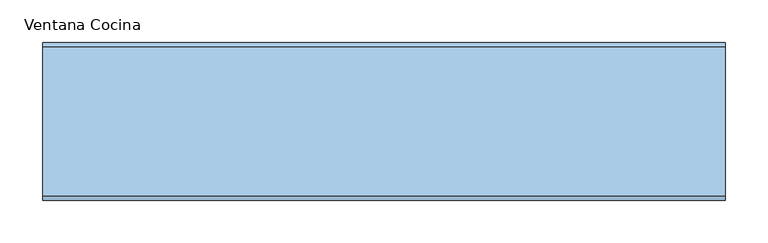
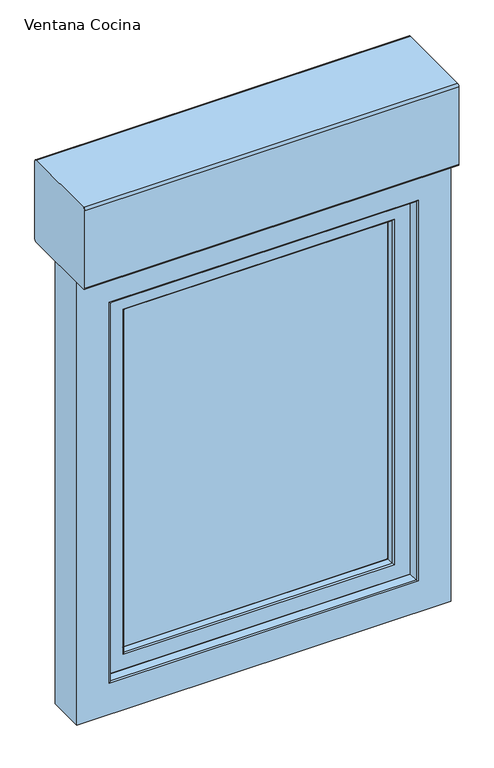
"""IFC4 building model written with IfcOpenShell, lengths in millimetres: window geometry, 2019_ES_Ventana_Replus_re80pvc301_10100_box_1-Hoja_con-Compacto : Ventana Cocina."""

from ifc_helpers import new_model, si_unit, point, frame, frame_2d, origin, place, context, project, spatial, polyline, circle_curve, ellipse_curve, trimmed, segment, composite_curve, outline, extrude, source, transform, mapped, element, save
from ifc_brep_helpers import plane_surface, cylinder_surface, advanced_brep


def ventana_cocina_4c5644c3(model_context):
    return source(origin(), model_context, "Body", "SolidModel", [
        extrude(outline(composite_curve([segment(trimmed(circle_curve(frame_2d((-55.0, 1815.0)), 5.0), [point((-55.0, 1810.0))], [point((-60.0, 1815.0))], False, "CARTESIAN"), True, "CONTINUOUS"), segment(polyline([(-60.0, 1815.0), (-60.0, 1990.0)]), True, "CONTINUOUS"), segment(trimmed(circle_curve(frame_2d((-55.0, 1990.0)), 5.0), [point((-60.0, 1990.0))], [point((-55.0, 1995.0))], False, "CARTESIAN"), True, "CONTINUOUS"), segment(polyline([(-55.0, 1995.0), (120.0, 1995.0)]), True, "CONTINUOUS"), segment(trimmed(circle_curve(frame_2d((120.0, 1990.0)), 5.0), [point((120.0, 1995.0))], [point((125.0, 1990.0))], False, "CARTESIAN"), True, "CONTINUOUS"), segment(polyline([(125.0, 1990.0), (125.0, 1815.0)]), True, "CONTINUOUS"), segment(trimmed(circle_curve(frame_2d((120.0, 1815.0)), 5.0), [point((125.0, 1815.0))], [point((120.0, 1810.0))], False, "CARTESIAN"), True, "CONTINUOUS"), segment(polyline([(120.0, 1810.0), (-55.0, 1810.0)]), True, "CONTINUOUS")], self_intersect=False)), frame((-400.0, 0.0, 0.0), z_axis=(1.0, 0.0, 0.0), x_axis=(0.0, 1.0, 0.0)), (0.0, 0.0, 1.0), 800.0),
        extrude(outline(polyline([(78.4999991, 1470.0), (118.4999991, 1470.0), (118.4999991, 1360.0), (98.4999991, 1360.0), (98.4999991, 1450.0), (78.4999991, 1450.0), (78.4999991, 1470.0)])), frame((-334.1999993, 0.0, 0.0), z_axis=(1.0, 0.0, 0.0), x_axis=(0.0, 1.0, 0.0)), (0.0, 0.0, 1.0), 12.0),
        extrude(outline(polyline([(-313.9687607, 78.4999991), (-313.9687607, 68.4999991), (-342.4312378, 68.4999991), (-342.4312378, 78.4999991), (-313.9687607, 78.4999991)])), frame((0.0, 0.0, 1435.217127), z_axis=(0.0, 0.0, 1.0), x_axis=(1.0, 0.0, 0.0)), (0.0, 0.0, 1.0), 49.565746),
        extrude(outline(polyline([(909.8, 297.1999993), (1707.2, 297.1999993), (1707.2, -297.1999993), (909.8, -297.1999993), (909.8, 297.1999993)]), holes=[polyline([(1699.2, 289.1999993), (917.8, 289.1999993), (917.8, -289.1999993), (1699.2, -289.1999993), (1699.2, 289.1999993)])]), frame((0.0, 10.9999999, 0.0), z_axis=(0.0, 1.0, 0.0), x_axis=(0.0, 0.0, 1.0)), (0.0, 0.0, 1.0), 16.0),
        extrude(outline(polyline([(909.8131934, 297.1868058), (1707.1868066, 297.1868058), (1707.1868066, -297.1868058), (909.8131934, -297.1868058), (909.8131934, 297.1868058)]), holes=[polyline([(1699.2, 289.1999993), (917.8, 289.1999993), (917.8, -289.1999993), (1699.2, -289.1999993), (1699.2, 289.1999993)])]), frame((0.0, 31.0000001, 0.0), z_axis=(0.0, 1.0, 0.0), x_axis=(0.0, 0.0, 1.0)), (0.0, 0.0, 1.0), 16.0),
        extrude(outline(polyline([(297.1999993, 6.9999997), (-297.1999993, 6.9999997), (-297.1999993, 10.9999999), (297.1999993, 10.9999999), (297.1999993, 6.9999997)])), frame((0.0, 0.0, 903.7946451), z_axis=(0.0, 0.0, 1.0), x_axis=(1.0, 0.0, 0.0)), (0.0, 0.0, 1.0), 809.4053549),
        extrude(outline(polyline([(297.1999993, 26.9999999), (-297.1999993, 26.9999999), (-297.1999993, 31.0000001), (297.1999993, 31.0000001), (297.1999993, 26.9999999)])), frame((0.0, 0.0, 903.7946451), z_axis=(0.0, 0.0, 1.0), x_axis=(1.0, 0.0, 0.0)), (0.0, 0.0, 1.0), 809.4053549),
        extrude(outline(polyline([(297.1999993, 47.0000001), (-297.1999993, 47.0000001), (-297.1999993, 51.0000003), (297.1999993, 51.0000003), (297.1999993, 47.0000001)])), frame((0.0, 0.0, 903.7946451), z_axis=(0.0, 0.0, 1.0), x_axis=(1.0, 0.0, 0.0)), (0.0, 0.0, 1.0), 809.4053549),
        advanced_brep(
        [(287.2913171, -9.2764571, 1697.2913178), (287.2913171, -9.2764571, 922.7086822), (290.1890946, -11.5, 919.8109047), (290.1890946, -11.5, 1700.1890953), (330.1999993, -11.5, 879.8), (330.1999993, -11.5, 1740.2), (-330.1999993, -11.5, 1740.2), (-330.1999993, -11.5, 879.8), (-290.1890946, -11.5, 919.8109047), (-290.1890946, -11.5, 1700.1890953), (-287.2913171, -9.2764571, 922.7086822), (284.1757968, 2.3508228, 1694.1757976), (284.1757968, 2.3508228, 925.8242024), (-284.1757968, 2.3508228, 925.8242024), (284.6739305, 3.0000033, 1694.6739313), (284.6739305, 3.0000033, 925.3260687), (-284.6739305, 3.0000033, 925.3260687), (291.1999993, 3.0000033, 1701.2), (291.1999993, 3.0000033, 918.8), (-291.1999993, 3.0000033, 918.8), (-291.1999993, 3.0000033, 1701.2), (-284.6739305, 3.0000033, 1694.6739313), (291.1999993, 6.9999997, 1701.2), (291.1999993, 6.9999997, 918.8), (-291.1999993, 6.9999997, 918.8), (311.8162192, 6.9999997, 1721.8162199), (311.8162192, 6.9999997, 898.1837801), (-311.8162192, 6.9999997, 898.1837801), (-311.8162192, 6.9999997, 1721.8162199), (-291.1999993, 6.9999997, 1701.2), (309.1999993, 25.6153717, 1719.2), (309.1999993, 25.6153717, 900.8), (-309.1999993, 25.6153717, 900.8), (309.1999993, 56.4999995, 1719.2), (309.1999993, 56.4999995, 900.8), (-309.1999993, 56.4999995, 900.8), (-309.1999993, 56.4999995, 1719.2), (297.1999993, 56.4999995, 1707.2), (297.1999993, 56.4999995, 912.8), (-297.1999993, 56.4999995, 912.8), (-297.1999993, 56.4999995, 1707.2), (297.1999993, 51.0000003, 1707.2), (297.1999993, 51.0000003, 912.8), (-297.1999993, 51.0000003, 912.8), (-297.1999993, 51.0000003, 1707.2), (286.007687, 51.0000003, 1696.0076877), (286.007687, 51.0000003, 923.9923123), (-286.007687, 51.0000003, 923.9923123), (-286.007687, 51.0000003, 1696.0076877), (285.4940999, 51.6693201, 1695.4941006), (285.4940999, 51.6693201, 924.5058994), (-285.4940999, 51.6693201, 924.5058994), (288.8993918, 64.3780426, 1698.8993925), (288.8993918, 64.3780426, 921.1006075), (-288.8993918, 64.3780426, 921.1006075), (292.6234971, 67.3403297, 1702.6234978), (292.6234971, 67.3403297, 917.3765022), (-292.6234971, 67.3403297, 917.3765022), (305.6488427, 67.7951848, 1715.6488434), (305.6488427, 67.7951848, 904.3511566), (-305.6488427, 67.7951848, 904.3511566), (306.1999993, 67.2629391, 1716.2), (306.1999993, 67.2629391, 903.8), (-306.1999993, 67.2629391, 903.8), (307.4370593, 68.4999991, 1717.43706), (307.4370593, 68.4999991, 902.56294), (-307.4370593, 68.4999991, 902.56294), (360.1999993, 68.4999991, 1770.2), (360.1999993, 68.4999991, 849.8), (-360.1999993, 68.4999991, 849.8), (-360.1999993, 68.4999991, 1770.2), (-307.4370593, 68.4999991, 1717.43706), (363.1999993, 65.4999991, 1773.2), (363.1999993, 65.4999991, 846.8), (-363.1999993, 65.4999991, 846.8), (363.1999993, 50.0, 1773.2), (363.1999993, 50.0, 846.8), (-363.1999993, 50.0, 846.8), (-363.1999993, 50.0, 1773.2), (343.1999993, 50.0, 1753.2), (343.1999993, 50.0, 866.8), (-343.1999993, 50.0, 866.8), (-343.1999993, 50.0, 1753.2), (343.1999993, 11.9999991, 1753.2), (343.1999993, 11.9999991, 866.8), (-343.1999993, 11.9999991, 866.8), (-343.1999993, 11.9999991, 1753.2), (330.1999993, 11.9999991, 1740.2), (330.1999993, 11.9999991, 879.8), (-330.1999993, 11.9999991, 879.8), (-330.1999993, 11.9999991, 1740.2), (-287.2913171, -9.2764571, 1697.2913178), (-284.1757968, 2.3508228, 1694.1757976), (-309.1999993, 25.6153717, 1719.2), (-285.4940999, 51.6693201, 1695.4941006), (-288.8993918, 64.3780426, 1698.8993925), (-292.6234971, 67.3403297, 1702.6234978), (-305.6488427, 67.7951848, 1715.6488434), (-306.1999993, 67.2629391, 1716.2), (-363.1999993, 65.4999991, 1773.2)],
        [
            (0, 1),
            (1, 2, ellipse_curve(frame((290.1890946, -8.5, 919.8109047), z_axis=(0.7071067811865475, 0.0, 0.7071067811865475), x_axis=(-0.7071067811865474, 0.0, 0.7071067811865476)), 4.2426407, 3.0)),
            (2, 3),
            (3, 0, ellipse_curve(frame((290.1890946, -8.5, 1700.1890953), z_axis=(0.7071067811865475, 0.0, -0.7071067811865475), x_axis=(0.7071067811865474, 0.0, 0.7071067811865476)), 4.2426407, 3.0)),
            (4, 5),
            (5, 6),
            (6, 7),
            (7, 4),
            (2, 8),
            (8, 9),
            (9, 3),
            (1, 10),
            (10, 8, ellipse_curve(frame((-290.1890946, -8.5, 919.8109047), z_axis=(0.7071067811865475, 0.0, -0.7071067811865475), x_axis=(0.7071067811865476, 0.0, 0.7071067811865474)), 4.2426407, 3.0)),
            (11, 12),
            (12, 1),
            (0, 11),
            (12, 13),
            (13, 10),
            (14, 15),
            (15, 12, ellipse_curve(frame((284.6739305, 2.4842973, 925.3260687), z_axis=(0.7071067811865475, 0.0, 0.7071067811865475), x_axis=(-0.7071067811865474, 0.0, 0.7071067811865476)), 0.7293184, 0.515706)),
            (11, 14, ellipse_curve(frame((284.6739305, 2.4842973, 1694.6739313), z_axis=(0.7071067811865475, 0.0, -0.7071067811865475), x_axis=(0.7071067811865474, 0.0, 0.7071067811865476)), 0.7293184, 0.515706)),
            (15, 16),
            (16, 13, ellipse_curve(frame((-284.6739305, 2.4842973, 925.3260687), z_axis=(0.7071067811865475, 0.0, -0.7071067811865475), x_axis=(0.7071067811865476, 0.0, 0.7071067811865474)), 0.7293184, 0.515706)),
            (17, 18),
            (18, 19),
            (19, 20),
            (20, 17),
            (14, 21),
            (21, 16),
            (22, 23),
            (23, 18),
            (17, 22),
            (23, 24),
            (24, 19),
            (25, 26),
            (26, 27),
            (27, 28),
            (28, 25),
            (22, 29),
            (29, 24),
            (30, 31),
            (31, 26),
            (25, 30),
            (31, 32),
            (32, 27),
            (33, 34),
            (34, 31),
            (30, 33),
            (34, 35),
            (35, 32),
            (33, 36),
            (36, 35),
            (37, 38),
            (38, 39),
            (39, 40),
            (40, 37),
            (41, 42),
            (42, 38),
            (37, 41),
            (42, 43),
            (43, 39),
            (41, 44),
            (44, 43),
            (45, 46),
            (46, 47),
            (47, 48),
            (48, 45),
            (49, 50),
            (50, 46, ellipse_curve(frame((286.007687, 51.5317048, 923.9923123), z_axis=(0.7071067811865475, 0.0, 0.7071067811865475), x_axis=(-0.7071067811865474, 0.0, 0.7071067811865476)), 0.7519437, 0.5317045)),
            (45, 49, ellipse_curve(frame((286.007687, 51.5317048, 1696.0076877), z_axis=(0.7071067811865475, 0.0, -0.7071067811865475), x_axis=(0.7071067811865474, 0.0, 0.7071067811865476)), 0.7519437, 0.5317045)),
            (50, 51),
            (51, 47, ellipse_curve(frame((-286.007687, 51.5317048, 923.9923123), z_axis=(0.7071067811865475, 0.0, -0.7071067811865475), x_axis=(0.7071067811865476, 0.0, 0.7071067811865474)), 0.7519437, 0.5317045)),
            (52, 53),
            (53, 50),
            (49, 52),
            (53, 54),
            (54, 51),
            (55, 56),
            (56, 53, ellipse_curve(frame((292.7630951, 63.3427664, 917.2369042), z_axis=(0.7071067811865475, 0.0, 0.7071067811865475), x_axis=(-0.7071067811865474, 0.0, 0.7071067811865476)), 5.6568542, 4.0)),
            (52, 55, ellipse_curve(frame((292.7630951, 63.3427664, 1702.7630958), z_axis=(0.7071067811865475, 0.0, -0.7071067811865475), x_axis=(0.7071067811865474, 0.0, 0.7071067811865476)), 5.6568542, 4.0)),
            (56, 57),
            (57, 54, ellipse_curve(frame((-292.7630951, 63.3427664, 917.2369042), z_axis=(0.7071067811865475, 0.0, -0.7071067811865475), x_axis=(0.7071067811865476, 0.0, 0.7071067811865474)), 5.6568542, 4.0)),
            (58, 59),
            (59, 56),
            (55, 58),
            (59, 60),
            (60, 57),
            (61, 62),
            (62, 59, ellipse_curve(frame((305.6674291, 67.2629391, 904.3325701), z_axis=(0.7071067811865475, 0.0, 0.7071067811865475), x_axis=(-0.7071067811865474, 0.0, 0.7071067811865476)), 0.7531679, 0.5325701)),
            (58, 61, ellipse_curve(frame((305.6674291, 67.2629391, 1715.6674299), z_axis=(0.7071067811865475, 0.0, -0.7071067811865475), x_axis=(0.7071067811865474, 0.0, 0.7071067811865476)), 0.7531679, 0.5325701)),
            (62, 63),
            (63, 60, ellipse_curve(frame((-305.6674291, 67.2629391, 904.3325701), z_axis=(0.7071067811865475, 0.0, -0.7071067811865475), x_axis=(0.7071067811865476, 0.0, 0.7071067811865474)), 0.7531679, 0.5325701)),
            (64, 65),
            (65, 62, ellipse_curve(frame((307.4370593, 67.2629391, 902.56294), z_axis=(0.7071067811865475, 0.0, 0.7071067811865475), x_axis=(-0.7071067811865474, 0.0, 0.7071067811865476)), 1.7494671, 1.23706)),
            (61, 64, ellipse_curve(frame((307.4370593, 67.2629391, 1717.43706), z_axis=(0.7071067811865475, 0.0, -0.7071067811865475), x_axis=(0.7071067811865474, 0.0, 0.7071067811865476)), 1.7494671, 1.23706)),
            (65, 66),
            (66, 63, ellipse_curve(frame((-307.4370593, 67.2629391, 902.56294), z_axis=(0.7071067811865475, 0.0, -0.7071067811865475), x_axis=(0.7071067811865476, 0.0, 0.7071067811865474)), 1.7494671, 1.23706)),
            (67, 68),
            (68, 69),
            (69, 70),
            (70, 67),
            (64, 71),
            (71, 66),
            (72, 73),
            (73, 68, ellipse_curve(frame((360.1999993, 65.4999991, 849.8), z_axis=(0.7071067811865475, 0.0, 0.7071067811865475), x_axis=(-0.7071067811865474, 0.0, 0.7071067811865476)), 4.2426407, 3.0)),
            (67, 72, ellipse_curve(frame((360.1999993, 65.4999991, 1770.2), z_axis=(0.7071067811865475, 0.0, -0.7071067811865475), x_axis=(0.7071067811865474, 0.0, 0.7071067811865476)), 4.2426407, 3.0)),
            (73, 74),
            (74, 69, ellipse_curve(frame((-360.1999993, 65.4999991, 849.8), z_axis=(0.7071067811865475, 0.0, -0.7071067811865475), x_axis=(0.7071067811865476, 0.0, 0.7071067811865474)), 4.2426407, 3.0)),
            (75, 76),
            (76, 73),
            (72, 75),
            (76, 77),
            (77, 74),
            (75, 78),
            (78, 77),
            (79, 80),
            (80, 81),
            (81, 82),
            (82, 79),
            (79, 83),
            (83, 84),
            (84, 80),
            (84, 85),
            (85, 81),
            (83, 86),
            (86, 85),
            (87, 88),
            (88, 89),
            (89, 90),
            (90, 87),
            (87, 5),
            (4, 88),
            (7, 89),
            (10, 91),
            (91, 9, ellipse_curve(frame((-290.1890946, -8.5, 1700.1890953), z_axis=(-0.7071067811865475, 0.0, -0.7071067811865475), x_axis=(0.7071067811865474, 0.0, -0.7071067811865476)), 4.2426407, 3.0)),
            (13, 92),
            (92, 91),
            (21, 92, ellipse_curve(frame((-284.6739305, 2.4842973, 1694.6739313), z_axis=(-0.7071067811865475, 0.0, -0.7071067811865475), x_axis=(0.7071067811865474, 0.0, -0.7071067811865476)), 0.7293184, 0.515706)),
            (29, 20),
            (32, 93),
            (93, 28),
            (36, 93),
            (44, 40),
            (51, 94),
            (94, 48, ellipse_curve(frame((-286.007687, 51.5317048, 1696.0076877), z_axis=(-0.7071067811865475, 0.0, -0.7071067811865475), x_axis=(0.7071067811865474, 0.0, -0.7071067811865476)), 0.7519437, 0.5317045)),
            (54, 95),
            (95, 94),
            (57, 96),
            (96, 95, ellipse_curve(frame((-292.7630951, 63.3427664, 1702.7630958), z_axis=(-0.7071067811865475, 0.0, -0.7071067811865475), x_axis=(0.7071067811865474, 0.0, -0.7071067811865476)), 5.6568542, 4.0)),
            (60, 97),
            (97, 96),
            (63, 98),
            (98, 97, ellipse_curve(frame((-305.6674291, 67.2629391, 1715.6674299), z_axis=(-0.7071067811865475, 0.0, -0.7071067811865475), x_axis=(0.7071067811865474, 0.0, -0.7071067811865476)), 0.7531679, 0.5325701)),
            (71, 98, ellipse_curve(frame((-307.4370593, 67.2629391, 1717.43706), z_axis=(-0.7071067811865475, 0.0, -0.7071067811865475), x_axis=(0.7071067811865474, 0.0, -0.7071067811865476)), 1.7494671, 1.23706)),
            (74, 99),
            (99, 70, ellipse_curve(frame((-360.1999993, 65.4999991, 1770.2), z_axis=(-0.7071067811865475, 0.0, -0.7071067811865475), x_axis=(0.7071067811865474, 0.0, -0.7071067811865476)), 4.2426407, 3.0)),
            (78, 99),
            (86, 82),
            (6, 90),
            (91, 0),
            (92, 11),
            (93, 30),
            (94, 49),
            (95, 52),
            (96, 55),
            (97, 58),
            (98, 61),
            (99, 72),
        ],
        [
            cylinder_surface(frame((290.1890946, -8.5, 1773.2), z_axis=(0.0, 0.0, 1.0), x_axis=(-1.0, 0.0, 0.0)), 3.0),
            plane_surface(frame((-330.1999993, -11.5, 1740.2), z_axis=(0.0, -1.0, 0.0), x_axis=(1.0, 0.0, 0.0))),
            cylinder_surface(frame((363.1999993, -8.5, 919.8109047), z_axis=(1.0, 0.0, 0.0), x_axis=(0.0, 0.0, 1.0)), 3.0),
            plane_surface(frame((287.2913171, -9.2764571, 1697.2913178), z_axis=(-0.9659258263570556, -0.258819044848789, 0.0), x_axis=(0.0, 0.0, -1.0))),
            plane_surface(frame((287.2913171, -9.2764571, 922.7086822), z_axis=(0.0, -0.2588190448487859, 0.9659258263570565), x_axis=(-1.0, 0.0, 0.0))),
            cylinder_surface(frame((284.6739305, 2.4842973, 1773.2), z_axis=(0.0, 0.0, 1.0), x_axis=(-1.0, 0.0, 0.0)), 0.515706),
            cylinder_surface(frame((363.1999993, 2.4842973, 925.3260687), z_axis=(1.0, 0.0, 0.0), x_axis=(0.0, 0.0, 1.0)), 0.515706),
            plane_surface(frame((-284.6739305, 3.0000033, 1694.6739313), z_axis=(0.0, 1.0, 0.0), x_axis=(1.0, 0.0, 0.0))),
            plane_surface(frame((291.1999993, 3.0000033, 1701.2), z_axis=(-1.0, 0.0, 0.0), x_axis=(0.0, 0.0, -1.0))),
            plane_surface(frame((291.1999993, 3.0000033, 918.8), z_axis=(0.0, 0.0, 1.0), x_axis=(-1.0, 0.0, 0.0))),
            plane_surface(frame((-291.1999993, 6.9999997, 1701.2), z_axis=(0.0, 1.0, 0.0), x_axis=(1.0, 0.0, 0.0))),
            plane_surface(frame((311.8162192, 6.9999997, 1721.8162199), z_axis=(-0.9902680687415736, -0.13917310096004265, 0.0), x_axis=(0.0, 0.0, -1.0))),
            plane_surface(frame((311.8162192, 6.9999997, 898.1837801), z_axis=(0.0, -0.13917310096003943, 0.990268068741574), x_axis=(-1.0, 0.0, 0.0))),
            plane_surface(frame((309.1999993, 25.6153717, 1719.2), z_axis=(-1.0, 0.0, 0.0), x_axis=(0.0, 0.0, -1.0))),
            plane_surface(frame((309.1999993, 25.6153717, 900.8), z_axis=(0.0, 0.0, 1.0), x_axis=(-1.0, 0.0, 0.0))),
            plane_surface(frame((-309.1999993, 56.4999995, 1719.2), z_axis=(0.0, -1.0, 0.0), x_axis=(1.0, 0.0, 0.0))),
            plane_surface(frame((297.1999993, 56.4999995, 1707.2), z_axis=(1.0, 0.0, 0.0), x_axis=(0.0, 0.0, -1.0))),
            plane_surface(frame((297.1999993, 56.4999995, 912.8), z_axis=(0.0, 0.0, -1.0), x_axis=(-1.0, 0.0, 0.0))),
            plane_surface(frame((-297.1999993, 51.0000003, 1707.2), z_axis=(0.0, -1.0, 0.0), x_axis=(1.0, 0.0, 0.0))),
            cylinder_surface(frame((286.007687, 51.5317048, 1773.2), z_axis=(0.0, 0.0, 1.0), x_axis=(-1.0, 0.0, 0.0)), 0.5317045),
            cylinder_surface(frame((363.1999993, 51.5317048, 923.9923123), z_axis=(1.0, 0.0, 0.0), x_axis=(0.0, 0.0, 1.0)), 0.5317045),
            plane_surface(frame((285.4940999, 51.6693201, 1695.4941006), z_axis=(-0.9659258262890666, 0.2588190451025272, 0.0), x_axis=(0.0, 0.0, -1.0))),
            plane_surface(frame((285.4940999, 51.6693201, 924.5058994), z_axis=(0.0, 0.2588190451025303, 0.9659258262890658), x_axis=(-1.0, 0.0, 0.0))),
            cylinder_surface(frame((292.7630951, 63.3427664, 1773.2), z_axis=(0.0, 0.0, 1.0), x_axis=(-1.0, 0.0, 0.0)), 4.0),
            cylinder_surface(frame((363.1999993, 63.3427664, 917.2369042), z_axis=(1.0, 0.0, 0.0), x_axis=(0.0, 0.0, 1.0)), 4.0),
            plane_surface(frame((292.6234971, 67.3403297, 1702.6234978), z_axis=(-0.03489949670250791, 0.9993908270190955, 0.0), x_axis=(0.0, 0.0, -1.0))),
            plane_surface(frame((292.6234971, 67.3403297, 917.3765022), z_axis=(0.0, 0.9993908270190957, 0.034899496702504675), x_axis=(-1.0, 0.0, 0.0))),
            cylinder_surface(frame((305.6674291, 67.2629391, 1773.2), z_axis=(0.0, 0.0, 1.0), x_axis=(-1.0, 0.0, 0.0)), 0.5325701),
            cylinder_surface(frame((363.1999993, 67.2629391, 904.3325701), z_axis=(1.0, 0.0, 0.0), x_axis=(0.0, 0.0, 1.0)), 0.5325701),
            cylinder_surface(frame((307.4370593, 67.2629391, 1773.2), z_axis=(0.0, 0.0, 1.0), x_axis=(-1.0, 0.0, 0.0)), 1.23706),
            cylinder_surface(frame((363.1999993, 67.2629391, 902.56294), z_axis=(1.0, 0.0, 0.0), x_axis=(0.0, 0.0, 1.0)), 1.23706),
            plane_surface(frame((-307.4370593, 68.4999991, 1717.43706), z_axis=(0.0, 1.0, 0.0), x_axis=(1.0, 0.0, 0.0))),
            cylinder_surface(frame((360.1999993, 65.4999991, 1773.2), z_axis=(0.0, 0.0, 1.0), x_axis=(-1.0, 0.0, 0.0)), 3.0),
            cylinder_surface(frame((363.1999993, 65.4999991, 849.8), z_axis=(1.0, 0.0, 0.0), x_axis=(0.0, 0.0, 1.0)), 3.0),
            plane_surface(frame((363.1999993, 65.4999991, 1773.2), z_axis=(1.0, 0.0, 0.0), x_axis=(0.0, 0.0, -1.0))),
            plane_surface(frame((363.1999993, 65.4999991, 846.8), z_axis=(0.0, 0.0, -1.0), x_axis=(-1.0, 0.0, 0.0))),
            plane_surface(frame((-359.2000019, 50.0, 1769.2000027), z_axis=(0.0, -1.0, 0.0), x_axis=(1.0, 0.0, 0.0))),
            plane_surface(frame((343.1999993, 45.0999991, 1753.2), z_axis=(1.0, 0.0, 0.0), x_axis=(0.0, 0.0, -1.0))),
            plane_surface(frame((343.1999993, 45.0999991, 866.8), z_axis=(0.0, 0.0, -1.0), x_axis=(-1.0, 0.0, 0.0))),
            plane_surface(frame((-335.7000002, 11.9999991, 1745.7000009), z_axis=(0.0, -1.0, 0.0), x_axis=(1.0, 0.0, 0.0))),
            plane_surface(frame((330.1999993, 1.4999991, 1740.2), z_axis=(1.0, 0.0, 0.0), x_axis=(0.0, 0.0, -1.0))),
            plane_surface(frame((330.1999993, 1.4999991, 879.8), z_axis=(0.0, 0.0, -1.0), x_axis=(-1.0, 0.0, 0.0))),
            cylinder_surface(frame((-290.1890946, -8.5, 846.8), z_axis=(0.0, 0.0, -1.0), x_axis=(1.0, 0.0, 0.0)), 3.0),
            plane_surface(frame((-287.2913171, -9.2764571, 922.7086822), z_axis=(0.9659258263570573, -0.25881904484878276, 0.0), x_axis=(0.0, 0.0, 1.0))),
            cylinder_surface(frame((-284.6739305, 2.4842973, 846.8), z_axis=(0.0, 0.0, -1.0), x_axis=(1.0, 0.0, 0.0)), 0.515706),
            plane_surface(frame((-291.1999993, 3.0000033, 918.8), z_axis=(1.0, 0.0, 0.0), x_axis=(0.0, 0.0, 1.0))),
            plane_surface(frame((-311.8162192, 6.9999997, 898.1837801), z_axis=(0.9902680687415745, -0.1391731009600362, 0.0), x_axis=(0.0, 0.0, 1.0))),
            plane_surface(frame((-309.1999993, 25.6153717, 900.8), z_axis=(1.0, 0.0, 0.0), x_axis=(0.0, 0.0, 1.0))),
            plane_surface(frame((-297.1999993, 56.4999995, 912.8), z_axis=(-1.0, 0.0, 0.0), x_axis=(0.0, 0.0, 1.0))),
            cylinder_surface(frame((-286.007687, 51.5317048, 846.8), z_axis=(0.0, 0.0, -1.0), x_axis=(1.0, 0.0, 0.0)), 0.5317045),
            plane_surface(frame((-285.4940999, 51.6693201, 924.5058994), z_axis=(0.9659258262890649, 0.2588190451025334, 0.0), x_axis=(0.0, 0.0, 1.0))),
            cylinder_surface(frame((-292.7630951, 63.3427664, 846.8), z_axis=(0.0, 0.0, -1.0), x_axis=(1.0, 0.0, 0.0)), 4.0),
            plane_surface(frame((-292.6234971, 67.3403297, 917.3765022), z_axis=(0.03489949670250144, 0.9993908270190958, 0.0), x_axis=(0.0, 0.0, 1.0))),
            cylinder_surface(frame((-305.6674291, 67.2629391, 846.8), z_axis=(0.0, 0.0, -1.0), x_axis=(1.0, 0.0, 0.0)), 0.5325701),
            cylinder_surface(frame((-307.4370593, 67.2629391, 846.8), z_axis=(0.0, 0.0, -1.0), x_axis=(1.0, 0.0, 0.0)), 1.23706),
            cylinder_surface(frame((-360.1999993, 65.4999991, 846.8), z_axis=(0.0, 0.0, -1.0), x_axis=(1.0, 0.0, 0.0)), 3.0),
            plane_surface(frame((-363.1999993, 65.4999991, 846.8), z_axis=(-1.0, 0.0, 0.0), x_axis=(0.0, 0.0, 1.0))),
            plane_surface(frame((-343.1999993, 45.0999991, 866.8), z_axis=(-1.0, 0.0, 0.0), x_axis=(0.0, 0.0, 1.0))),
            plane_surface(frame((-330.1999993, 1.4999991, 879.8), z_axis=(-1.0, 0.0, 0.0), x_axis=(0.0, 0.0, 1.0))),
            cylinder_surface(frame((-363.1999993, -8.5, 1700.1890953), z_axis=(-1.0, 0.0, 0.0), x_axis=(0.0, 0.0, -1.0)), 3.0),
            plane_surface(frame((-287.2913171, -9.2764571, 1697.2913178), z_axis=(0.0, -0.2588190448487859, -0.9659258263570564), x_axis=(1.0, 0.0, 0.0))),
            cylinder_surface(frame((-363.1999993, 2.4842973, 1694.6739313), z_axis=(-1.0, 0.0, 0.0), x_axis=(0.0, 0.0, -1.0)), 0.515706),
            plane_surface(frame((-291.1999993, 3.0000033, 1701.2), z_axis=(0.0, 0.0, -1.0), x_axis=(1.0, 0.0, 0.0))),
            plane_surface(frame((-311.8162192, 6.9999997, 1721.8162199), z_axis=(0.0, -0.13917310096003943, -0.990268068741574), x_axis=(1.0, 0.0, 0.0))),
            plane_surface(frame((-309.1999993, 25.6153717, 1719.2), z_axis=(0.0, 0.0, -1.0), x_axis=(1.0, 0.0, 0.0))),
            plane_surface(frame((-297.1999993, 56.4999995, 1707.2), z_axis=(0.0, 0.0, 1.0), x_axis=(1.0, 0.0, 0.0))),
            cylinder_surface(frame((-363.1999993, 51.5317048, 1696.0076877), z_axis=(-1.0, 0.0, 0.0), x_axis=(0.0, 0.0, -1.0)), 0.5317045),
            plane_surface(frame((-285.4940999, 51.6693201, 1695.4941006), z_axis=(0.0, 0.2588190451025303, -0.9659258262890658), x_axis=(1.0, 0.0, 0.0))),
            cylinder_surface(frame((-363.1999993, 63.3427664, 1702.7630958), z_axis=(-1.0, 0.0, 0.0), x_axis=(0.0, 0.0, -1.0)), 4.0),
            plane_surface(frame((-292.6234971, 67.3403297, 1702.6234978), z_axis=(0.0, 0.9993908270190957, -0.034899496702504675), x_axis=(1.0, 0.0, 0.0))),
            cylinder_surface(frame((-363.1999993, 67.2629391, 1715.6674299), z_axis=(-1.0, 0.0, 0.0), x_axis=(0.0, 0.0, -1.0)), 0.5325701),
            cylinder_surface(frame((-363.1999993, 67.2629391, 1717.43706), z_axis=(-1.0, 0.0, 0.0), x_axis=(0.0, 0.0, -1.0)), 1.23706),
            cylinder_surface(frame((-363.1999993, 65.4999991, 1770.2), z_axis=(-1.0, 0.0, 0.0), x_axis=(0.0, 0.0, -1.0)), 3.0),
            plane_surface(frame((-363.1999993, 65.4999991, 1773.2), z_axis=(0.0, 0.0, 1.0), x_axis=(1.0, 0.0, 0.0))),
            plane_surface(frame((-343.1999993, 45.0999991, 1753.2), z_axis=(0.0, 0.0, 1.0), x_axis=(1.0, 0.0, 0.0))),
            plane_surface(frame((-330.1999993, 1.4999991, 1740.2), z_axis=(0.0, 0.0, 1.0), x_axis=(1.0, 0.0, 0.0))),
        ],
        [
            (0, [[1, 2, 3, 4]]),
            (1, [[5, 6, 7, 8], [-3, 9, 10, 11]]),
            (2, [[12, 13, -9, -2]]),
            (3, [[14, 15, -1, 16]]),
            (4, [[17, 18, -12, -15]]),
            (5, [[19, 20, -14, 21]]),
            (6, [[22, 23, -17, -20]]),
            (7, [[24, 25, 26, 27], [-19, 28, 29, -22]]),
            (8, [[30, 31, -24, 32]]),
            (9, [[33, 34, -25, -31]]),
            (10, [[35, 36, 37, 38], [-30, 39, 40, -33]]),
            (11, [[41, 42, -35, 43]]),
            (12, [[44, 45, -36, -42]]),
            (13, [[46, 47, -41, 48]]),
            (14, [[49, 50, -44, -47]]),
            (15, [[-46, 51, 52, -49], [53, 54, 55, 56]]),
            (16, [[57, 58, -53, 59]]),
            (17, [[60, 61, -54, -58]]),
            (18, [[-57, 62, 63, -60], [64, 65, 66, 67]]),
            (19, [[68, 69, -64, 70]]),
            (20, [[71, 72, -65, -69]]),
            (21, [[73, 74, -68, 75]]),
            (22, [[76, 77, -71, -74]]),
            (23, [[78, 79, -73, 80]]),
            (24, [[81, 82, -76, -79]]),
            (25, [[83, 84, -78, 85]]),
            (26, [[86, 87, -81, -84]]),
            (27, [[88, 89, -83, 90]]),
            (28, [[91, 92, -86, -89]]),
            (29, [[93, 94, -88, 95]]),
            (30, [[96, 97, -91, -94]]),
            (31, [[98, 99, 100, 101], [-93, 102, 103, -96]]),
            (32, [[104, 105, -98, 106]]),
            (33, [[107, 108, -99, -105]]),
            (34, [[109, 110, -104, 111]]),
            (35, [[112, 113, -107, -110]]),
            (36, [[-109, 114, 115, -112], [116, 117, 118, 119]]),
            (37, [[120, 121, 122, -116]]),
            (38, [[123, 124, -117, -122]]),
            (39, [[-121, 125, 126, -123], [127, 128, 129, 130]]),
            (40, [[131, -5, 132, -127]]),
            (41, [[-8, 133, -128, -132]]),
            (42, [[134, 135, -10, -13]]),
            (43, [[136, 137, -134, -18]]),
            (44, [[-29, 138, -136, -23]]),
            (45, [[-40, 139, -26, -34]]),
            (46, [[140, 141, -37, -45]]),
            (47, [[-52, 142, -140, -50]]),
            (48, [[-63, 143, -55, -61]]),
            (49, [[144, 145, -66, -72]]),
            (50, [[146, 147, -144, -77]]),
            (51, [[148, 149, -146, -82]]),
            (52, [[150, 151, -148, -87]]),
            (53, [[152, 153, -150, -92]]),
            (54, [[-103, 154, -152, -97]]),
            (55, [[155, 156, -100, -108]]),
            (56, [[-115, 157, -155, -113]]),
            (57, [[-126, 158, -118, -124]]),
            (58, [[-7, 159, -129, -133]]),
            (59, [[160, -4, -11, -135]]),
            (60, [[161, -16, -160, -137]]),
            (61, [[-28, -21, -161, -138]]),
            (62, [[-39, -32, -27, -139]]),
            (63, [[162, -43, -38, -141]]),
            (64, [[-51, -48, -162, -142]]),
            (65, [[-62, -59, -56, -143]]),
            (66, [[163, -70, -67, -145]]),
            (67, [[164, -75, -163, -147]]),
            (68, [[165, -80, -164, -149]]),
            (69, [[166, -85, -165, -151]]),
            (70, [[167, -90, -166, -153]]),
            (71, [[-102, -95, -167, -154]]),
            (72, [[168, -106, -101, -156]]),
            (73, [[-114, -111, -168, -157]]),
            (74, [[-125, -120, -119, -158]]),
            (75, [[-6, -131, -130, -159]]),
        ],
    ),
        advanced_brep(
        [(323.2673545, -12.758819, 1733.2673545), (323.2673545, -12.758819, 886.7326455), (327.2913185, -27.7764571, 882.7086815), (327.2913185, -27.7764571, 1737.2913185), (330.189096, -30.0, 879.810904), (330.189096, -30.0, 1740.189096), (-323.2673545, -12.758819, 886.7326455), (-327.2913185, -27.7764571, 882.7086815), (324.2332803, -11.5, 1734.2332803), (324.2332803, -11.5, 885.7667197), (400.0, -30.0, 1810.0), (400.0, -30.0, 810.0), (400.0, 50.0, 810.0), (400.0, 50.0, 1810.0), (-400.0, 50.0, 810.0), (-400.0, 50.0, 1810.0), (356.1999993, 50.0, 853.8000007), (356.1999993, 50.0, 1766.1999993), (-356.1999993, 50.0, 1766.1999993), (-356.1999993, 50.0, 853.8000007), (-400.0, -30.0, 810.0), (-400.0, -30.0, 1810.0), (-330.189096, -30.0, 879.810904), (-330.189096, -30.0, 1740.189096), (336.1891471, 8.0, 1746.1891471), (336.1891471, 8.0, 873.8108529), (336.1891471, -11.5, 873.8108529), (336.1891471, -11.5, 1746.1891471), (-336.1891471, -11.5, 873.8108529), (-336.1891471, -11.5, 1746.1891471), (-324.2332803, -11.5, 1734.2332803), (-324.2332803, -11.5, 885.7667197), (-336.1891471, 8.0, 873.8108529), (355.1999993, 8.0, 1765.1999993), (355.1999993, 8.0, 854.8000007), (-355.1999993, 8.0, 854.8000007), (-355.1999993, 8.0, 1765.1999993), (-336.1891471, 8.0, 1746.1891471), (355.1999993, 49.0, 854.8000007), (355.1999993, 49.0, 1765.1999993), (-355.1999993, 49.0, 854.8000007), (-323.2673545, -12.758819, 1733.2673545), (-327.2913185, -27.7764571, 1737.2913185), (-355.1999993, 49.0, 1765.1999993)],
        [
            (0, 1),
            (1, 2),
            (2, 3),
            (3, 0),
            (2, 4, ellipse_curve(frame((330.189096, -27.0, 879.810904), z_axis=(0.7071067811865475, 0.0, 0.7071067811865475), x_axis=(-0.7071067811865474, 0.0, 0.7071067811865476)), 4.2426407, 3.0)),
            (4, 5),
            (5, 3, ellipse_curve(frame((330.189096, -27.0, 1740.189096), z_axis=(0.7071067811865475, 0.0, -0.7071067811865475), x_axis=(0.7071067811865474, 0.0, 0.7071067811865476)), 4.2426407, 3.0)),
            (1, 6),
            (6, 7),
            (7, 2),
            (8, 9),
            (9, 1, ellipse_curve(frame((324.2332803, -12.5, 885.7667197), z_axis=(0.7071067811865475, 0.0, 0.7071067811865475), x_axis=(-0.7071067811865474, 0.0, 0.7071067811865476)), 1.4142136, 1.0)),
            (0, 8, ellipse_curve(frame((324.2332803, -12.5, 1734.2332803), z_axis=(0.7071067811865475, 0.0, -0.7071067811865475), x_axis=(0.7071067811865474, 0.0, 0.7071067811865476)), 1.4142136, 1.0)),
            (10, 11),
            (11, 12),
            (12, 13),
            (13, 10),
            (12, 14),
            (14, 15),
            (15, 13),
            (16, 17),
            (17, 18),
            (18, 19),
            (19, 16),
            (11, 20),
            (20, 14),
            (10, 21),
            (21, 20),
            (4, 22),
            (22, 23),
            (23, 5),
            (24, 25),
            (25, 26),
            (26, 27),
            (27, 24),
            (26, 28),
            (28, 29),
            (29, 27),
            (8, 30),
            (30, 31),
            (31, 9),
            (25, 32),
            (32, 28),
            (33, 34),
            (34, 35),
            (35, 36),
            (36, 33),
            (24, 37),
            (37, 32),
            (16, 38, ellipse_curve(frame((356.1999993, 49.0, 853.8000007), z_axis=(0.7071067811865475, 0.0, 0.7071067811865475), x_axis=(-0.7071067811865474, 0.0, 0.7071067811865476)), 1.4142136, 1.0)),
            (38, 39),
            (39, 17, ellipse_curve(frame((356.1999993, 49.0, 1766.1999993), z_axis=(0.7071067811865475, 0.0, -0.7071067811865475), x_axis=(0.7071067811865474, 0.0, 0.7071067811865476)), 1.4142136, 1.0)),
            (38, 34),
            (33, 39),
            (19, 40, ellipse_curve(frame((-356.1999993, 49.0, 853.8000007), z_axis=(0.7071067811865475, 0.0, -0.7071067811865475), x_axis=(0.7071067811865476, 0.0, 0.7071067811865474)), 1.4142136, 1.0)),
            (40, 38),
            (31, 6, ellipse_curve(frame((-324.2332803, -12.5, 885.7667197), z_axis=(0.7071067811865475, 0.0, -0.7071067811865475), x_axis=(0.7071067811865476, 0.0, 0.7071067811865474)), 1.4142136, 1.0)),
            (7, 22, ellipse_curve(frame((-330.189096, -27.0, 879.810904), z_axis=(0.7071067811865475, 0.0, -0.7071067811865475), x_axis=(0.7071067811865476, 0.0, 0.7071067811865474)), 4.2426407, 3.0)),
            (6, 41),
            (41, 42),
            (42, 7),
            (21, 15),
            (37, 29),
            (40, 35),
            (18, 43, ellipse_curve(frame((-356.1999993, 49.0, 1766.1999993), z_axis=(-0.7071067811865475, 0.0, -0.7071067811865475), x_axis=(0.7071067811865474, 0.0, -0.7071067811865476)), 1.4142136, 1.0)),
            (43, 40),
            (30, 41, ellipse_curve(frame((-324.2332803, -12.5, 1734.2332803), z_axis=(-0.7071067811865475, 0.0, -0.7071067811865475), x_axis=(0.7071067811865474, 0.0, -0.7071067811865476)), 1.4142136, 1.0)),
            (42, 23, ellipse_curve(frame((-330.189096, -27.0, 1740.189096), z_axis=(-0.7071067811865475, 0.0, -0.7071067811865475), x_axis=(0.7071067811865474, 0.0, -0.7071067811865476)), 4.2426407, 3.0)),
            (43, 36),
            (41, 0),
            (3, 42),
            (39, 43),
        ],
        [
            plane_surface(frame((327.2913185, -27.7764571, 1737.2913185), z_axis=(-0.9659258262890693, -0.25881904510251696, 0.0), x_axis=(0.0, 0.0, -1.0))),
            cylinder_surface(frame((330.189096, -27.0, 1810.0), z_axis=(0.0, 0.0, 1.0), x_axis=(-1.0, 0.0, 0.0)), 3.0),
            plane_surface(frame((327.2913185, -27.7764571, 882.7086815), z_axis=(0.0, -0.25881904510251386, 0.9659258262890702), x_axis=(-1.0, 0.0, 0.0))),
            cylinder_surface(frame((324.2332803, -12.5, 1810.0), z_axis=(0.0, 0.0, 1.0), x_axis=(-1.0, 0.0, 0.0)), 1.0),
            plane_surface(frame((400.0, 50.0, 1810.0), z_axis=(1.0, 0.0, 0.0), x_axis=(0.0, 0.0, -1.0))),
            plane_surface(frame((-356.1999993, 50.0, 1766.1999993), z_axis=(0.0, 1.0, 0.0), x_axis=(1.0, 0.0, 0.0))),
            plane_surface(frame((400.0, 50.0, 810.0), z_axis=(0.0, 0.0, -1.0), x_axis=(-1.0, 0.0, 0.0))),
            plane_surface(frame((-400.0, -30.0, 1810.0), z_axis=(0.0, -1.0, 0.0), x_axis=(1.0, 0.0, 0.0))),
            plane_surface(frame((336.1891471, -11.5, 1746.1891471), z_axis=(-1.0, 0.0, 0.0), x_axis=(0.0, 0.0, -1.0))),
            plane_surface(frame((-324.2332803, -11.5, 1734.2332803), z_axis=(0.0, 1.0, 0.0), x_axis=(1.0, 0.0, 0.0))),
            plane_surface(frame((336.1891471, -11.5, 873.8108529), z_axis=(0.0, 0.0, 1.0), x_axis=(-1.0, 0.0, 0.0))),
            plane_surface(frame((-336.1891471, 8.0, 1746.1891471), z_axis=(0.0, 1.0, 0.0), x_axis=(1.0, 0.0, 0.0))),
            cylinder_surface(frame((356.1999993, 49.0, 1810.0), z_axis=(0.0, 0.0, 1.0), x_axis=(-1.0, 0.0, 0.0)), 1.0),
            plane_surface(frame((355.1999993, 8.0, 1765.1999993), z_axis=(-1.0, 0.0, 0.0), x_axis=(0.0, 0.0, -1.0))),
            cylinder_surface(frame((400.0, 49.0, 853.8000007), z_axis=(1.0, 0.0, 0.0), x_axis=(0.0, 0.0, 1.0)), 1.0),
            cylinder_surface(frame((400.0, -12.5, 885.7667197), z_axis=(1.0, 0.0, 0.0), x_axis=(0.0, 0.0, 1.0)), 1.0),
            cylinder_surface(frame((400.0, -27.0, 879.810904), z_axis=(1.0, 0.0, 0.0), x_axis=(0.0, 0.0, 1.0)), 3.0),
            plane_surface(frame((-327.2913185, -27.7764571, 882.7086815), z_axis=(0.9659258262890711, -0.25881904510251075, 0.0), x_axis=(0.0, 0.0, 1.0))),
            plane_surface(frame((-400.0, 50.0, 810.0), z_axis=(-1.0, 0.0, 0.0), x_axis=(0.0, 0.0, 1.0))),
            plane_surface(frame((-336.1891471, -11.5, 873.8108529), z_axis=(1.0, 0.0, 0.0), x_axis=(0.0, 0.0, 1.0))),
            plane_surface(frame((355.1999993, 8.0, 854.8000007), z_axis=(0.0, 0.0, 1.0), x_axis=(-1.0, 0.0, 0.0))),
            cylinder_surface(frame((-356.1999993, 49.0, 810.0), z_axis=(0.0, 0.0, -1.0), x_axis=(1.0, 0.0, 0.0)), 1.0),
            cylinder_surface(frame((-324.2332803, -12.5, 810.0), z_axis=(0.0, 0.0, -1.0), x_axis=(1.0, 0.0, 0.0)), 1.0),
            cylinder_surface(frame((-330.189096, -27.0, 810.0), z_axis=(0.0, 0.0, -1.0), x_axis=(1.0, 0.0, 0.0)), 3.0),
            plane_surface(frame((-355.1999993, 8.0, 854.8000007), z_axis=(1.0, 0.0, 0.0), x_axis=(0.0, 0.0, 1.0))),
            plane_surface(frame((-327.2913185, -27.7764571, 1737.2913185), z_axis=(0.0, -0.25881904510251386, -0.9659258262890702), x_axis=(1.0, 0.0, 0.0))),
            plane_surface(frame((-400.0, 50.0, 1810.0), z_axis=(0.0, 0.0, 1.0), x_axis=(1.0, 0.0, 0.0))),
            plane_surface(frame((-336.1891471, -11.5, 1746.1891471), z_axis=(0.0, 0.0, -1.0), x_axis=(1.0, 0.0, 0.0))),
            cylinder_surface(frame((-400.0, 49.0, 1766.1999993), z_axis=(-1.0, 0.0, 0.0), x_axis=(0.0, 0.0, -1.0)), 1.0),
            cylinder_surface(frame((-400.0, -12.5, 1734.2332803), z_axis=(-1.0, 0.0, 0.0), x_axis=(0.0, 0.0, -1.0)), 1.0),
            cylinder_surface(frame((-400.0, -27.0, 1740.189096), z_axis=(-1.0, 0.0, 0.0), x_axis=(0.0, 0.0, -1.0)), 3.0),
            plane_surface(frame((-355.1999993, 8.0, 1765.1999993), z_axis=(0.0, 0.0, -1.0), x_axis=(1.0, 0.0, 0.0))),
        ],
        [
            (0, [[1, 2, 3, 4]]),
            (1, [[-3, 5, 6, 7]]),
            (2, [[8, 9, 10, -2]]),
            (3, [[11, 12, -1, 13]]),
            (4, [[14, 15, 16, 17]]),
            (5, [[-16, 18, 19, 20], [21, 22, 23, 24]]),
            (6, [[25, 26, -18, -15]]),
            (7, [[-14, 27, 28, -25], [-6, 29, 30, 31]]),
            (8, [[32, 33, 34, 35]]),
            (9, [[-34, 36, 37, 38], [-11, 39, 40, 41]]),
            (10, [[42, 43, -36, -33]]),
            (11, [[44, 45, 46, 47], [-32, 48, 49, -42]]),
            (12, [[-21, 50, 51, 52]]),
            (13, [[-51, 53, -44, 54]]),
            (14, [[-24, 55, 56, -50]]),
            (15, [[-41, 57, -8, -12]]),
            (16, [[-10, 58, -29, -5]]),
            (17, [[59, 60, 61, -9]]),
            (18, [[-28, 62, -19, -26]]),
            (19, [[-49, 63, -37, -43]]),
            (20, [[-56, 64, -45, -53]]),
            (21, [[-23, 65, 66, -55]]),
            (22, [[-40, 67, -59, -57]]),
            (23, [[-61, 68, -30, -58]]),
            (24, [[-66, 69, -46, -64]]),
            (25, [[70, -4, 71, -60]]),
            (26, [[-27, -17, -20, -62]]),
            (27, [[-48, -35, -38, -63]]),
            (28, [[-22, -52, 72, -65]]),
            (29, [[-39, -13, -70, -67]]),
            (30, [[-71, -7, -31, -68]]),
            (31, [[-72, -54, -47, -69]]),
        ],
    ),
    ])


if __name__ == "__main__":
    model = new_model("IFC4")
    model_context = context("Model", 3, world=origin())
    ifc_project = project(units=[si_unit("LENGTHUNIT", "METRE", prefix="MILLI")], contexts=[model_context])
    site = spatial("IfcSite", under=ifc_project)
    building = spatial("IfcBuilding", under=site)
    placement = place(None, origin())
    ventana_cocina_shape = ventana_cocina_4c5644c3(model_context)
    element("IfcWindow", 1, ObjectType="2019_ES_Ventana_Replus_re80pvc301_10100_box_1-Hoja_con-Compacto : Ventana Cocina", at=placement, inside=building, context=model_context, shape_type="MappedRepresentation", body=[
        mapped(ventana_cocina_shape, transform((0.0, 0.0, 0.0), x_axis=(1.0, 0.0, 0.0), y_axis=(0.0, 1.0, 0.0), z_axis=(0.0, 0.0, 1.0))),
    ])
    save(model, "model.ifc")

# Revit data of these elements
# Type "2019_ES_Ventana_Replus_re80pvc301_10100_box_1-Hoja_con-Compacto : Ventana Cocina"
#   Type Mark = "41"
#   URL = "https://replus.es/"
#   Product data url = "https://bimetica.com/es/objetos-bim-replus-ventana-practicable-oscilobatiente-una-hoja-con-compacto-9540"
#   Product Guid = ""
#   Model = "10100 BOX"
#   Material secondary = "Glass"
#   Material main = "PVC"
#   Manufacturer = "Replus"
#   Keynote = "08500"
#   EAN code = ""
#   Description = "Perfiles de PVC con triple junta (por junta rígida en el marco). Protegiendo de este modo todos los puntos de cierre y proporcionando una junta perimetral completa, con un grosor en el perfil de 3 mm. Vidrio de alta calidad con diferentes posibilidades"
#   Assembly Code = "B2020100"
#   Analytic Construction = "<None>"
#   Ι_Wll Thcknss [instance default] = 20.0 cm
#   Ι_Wdth Cntrl = 80.0 cm
#   Ι_Nst Cntrl [instance default] = 0.0 cm
#   Ι_Hndl Hght Cntrl = 65.0 cm
#   Ι_Hght Cntrl = 100.0 cm
#   Rough Width = 82.0 cm
#   Rough Height = 102.0 cm
#   Retranqueo [instance default] = 0.0 cm
#   I_Lf_Cntrl = 72.64 cm
#   Hueco = 1.0 cm
#   Height = 100.0 cm
#   Default Sill Height = 80.0 cm
#   Width = 80.0 cm
#   Altura de Manilla = 65.0 cm
#   Visibilidad Líneas Apertura - Planta = yes
#   Visibilidad Líneas Apertura - Alzado = yes
#   Exceso Dimensiones = no
#   Edition number = 1
#   Advertencia Dimensión = yes
#   Product Material = PVC - Replus - 9152 - White
#   Wall Closure = (empty or 0)
# Element 1 (IfcWindow, "2019_ES_Ventana_Replus_re80pvc301_10100_box_1-Hoja_con-Compacto : Ventana Cocina")
#   Ι_Wll Thcknss = 10.0 cm
#   Materials on its faces: "PVC - Replus - 9152 - White", "Rubber - Replus - Black", "Glass - Replus"
# Materials
#   "PVC - Replus - 9152 - White": class "Miscellaneous", colour RGB 174 174 166, transparency 0, Manufacturer = "Replus", Comments = "Rendering appearance not upgraded ", URL = "https://replus.es/", Cost = 0
#   "Rubber - Replus - Black": class "Plastic", colour RGB 63 63 63, transparency 0, Description = "Natural rubber, black", Cost = 0
#   "Glass - Replus": class "Glass", colour RGB 218 227 224, transparency 0.85, Cost = 0
